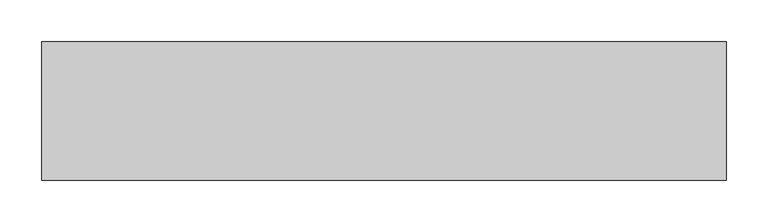
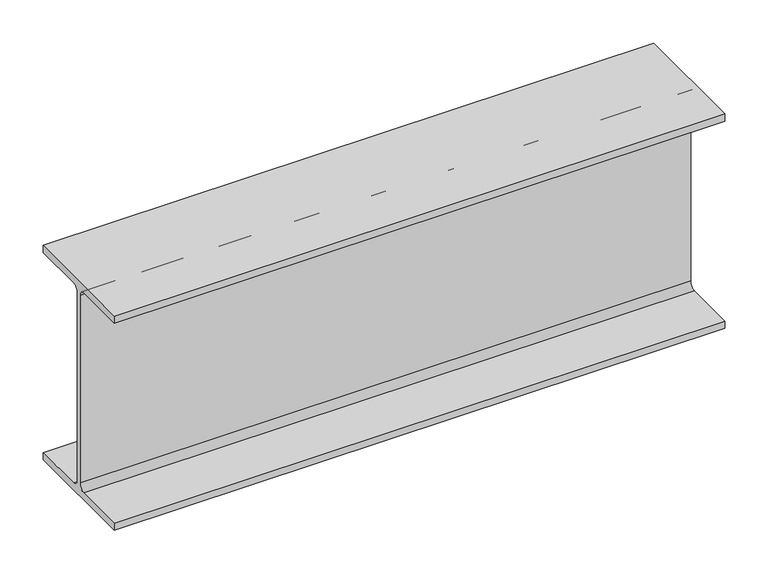
"""IFC4 building model written with IfcOpenShell, lengths in millimetres: beam geometry, Old_Steel Beam_H-KSD3502 : H_SB_ASB_H-390×300x10x16."""

import ifcopenshell
import ifcopenshell.guid

model = None  # the IFC model being written
_history = None  # IfcOwnerHistory: only IFC2X3 demands one
_inside = {}  # id of a spatial element -> (the spatial element, [elements in it])
_under = {}  # id of a project, library or spatial element -> (it, [spatial elements below it])
_declared = {}  # id of a project -> (the project, [libraries it declares])
_typed = {}  # id of a type object -> (the type object, [elements of that type])
_made_of = {}  # id of a material, layer set ... -> (it, [elements and type objects made of it])


def new_model(schema):
    """Start an empty IFC model of exactly this schema.

    Asked for "IFC4X3", IfcOpenShell would pick the latest addendum, in which some entities
    have other attributes; the version numbers below select the first issue.
    IFC2X3 requires an IfcOwnerHistory on every rooted entity: one is made here for all.
    """
    global model, _history
    if schema == "IFC4X3":
        model = ifcopenshell.file(schema_version=(4, 3, 0, 0))
    else:
        model = ifcopenshell.file(schema=schema)
    _inside.clear()
    _under.clear()
    _declared.clear()
    _typed.clear()
    _made_of.clear()
    _history = None
    if model.schema == "IFC2X3":
        org = make("IfcOrganization", Name="unknown")
        user = make(
            "IfcPersonAndOrganization",
            ThePerson=make("IfcPerson", FamilyName="unknown"),
            TheOrganization=org,
        )
        app = make(
            "IfcApplication",
            ApplicationDeveloper=org,
            Version="unknown",
            ApplicationFullName="unknown",
            ApplicationIdentifier="unknown",
        )
        _history = make(
            "IfcOwnerHistory",
            OwningUser=user,
            OwningApplication=app,
            ChangeAction="ADDED",
            CreationDate=0,
        )
    return model


def make(cls, **values):
    """One entity of the class cls with the attributes given. An attribute that is None is left unset."""
    return model.create_entity(
        cls, **{name: value for name, value in values.items() if value is not None}
    )


def rooted(cls, **values):
    """An entity with a GlobalId (a new one), such as an element, a storey or a relation."""
    return make(cls, GlobalId=ifcopenshell.guid.new(), OwnerHistory=_history, **values)


def si_unit(unit_type, name, prefix=None):
    """IfcSIUnit, for example si_unit("LENGTHUNIT", "METRE", prefix="MILLI")."""
    return make("IfcSIUnit", UnitType=unit_type, Prefix=prefix, Name=name)


def assignment(units):
    """IfcUnitAssignment: the units of a project."""
    return None if units is None else make("IfcUnitAssignment", Units=units)


def point(xyz):
    """IfcCartesianPoint."""
    return None if xyz is None else make("IfcCartesianPoint", Coordinates=xyz)


def direction(xyz):
    """IfcDirection."""
    return None if xyz is None else make("IfcDirection", DirectionRatios=xyz)


def frame(location, z_axis=None, x_axis=None):
    """IfcAxis2Placement3D, a coordinate frame: its origin and axes. An axis left out is left unset."""
    return make(
        "IfcAxis2Placement3D",
        Location=point(location),
        Axis=direction(z_axis),
        RefDirection=direction(x_axis),
    )


def frame_2d(location, x_axis=None):
    """IfcAxis2Placement2D, a coordinate frame in the plane: its origin and x axis."""
    return make(
        "IfcAxis2Placement2D", Location=point(location), RefDirection=direction(x_axis)
    )


def origin():
    """The frame at (0, 0, 0) with its axes left unset."""
    return frame((0.0, 0.0, 0.0))


def place(relative_to, where):
    """IfcLocalPlacement: puts the frame where relative to a parent placement (None: the world)."""
    return make(
        "IfcLocalPlacement", PlacementRelTo=relative_to, RelativePlacement=where
    )


def context(
    kind, dimensions, precision=None, world=None, true_north=None, identifier=None
):
    """IfcGeometricRepresentationContext, for example the 3D "Model" context."""
    return make(
        "IfcGeometricRepresentationContext",
        ContextIdentifier=identifier,
        ContextType=kind,
        CoordinateSpaceDimension=dimensions,
        Precision=precision,
        WorldCoordinateSystem=world,
        TrueNorth=true_north,
    )


def project(units=None, contexts=None):
    """IfcProject with its units and contexts."""
    return rooted(
        "IfcProject",
        Name="project",
        RepresentationContexts=contexts,
        UnitsInContext=assignment(units),
    )


def spatial(cls, under=None, at=None, **own):
    """A site, building, storey or space (cls), placed at a placement, below another one or the project."""
    s = rooted(cls, ObjectPlacement=at, **own)
    if under is not None:
        _under.setdefault(under.id(), (under, []))[1].append(s)
    return s


def polyline(points):
    """IfcPolyline through the points."""
    return make("IfcPolyline", Points=[point(p) for p in points])


def circle_curve(where, radius):
    """IfcCircle in the frame where."""
    return make("IfcCircle", Position=where, Radius=radius)


def trimmed(basis, trim1, trim2, sense, master):
    """IfcTrimmedCurve: the piece of a basis curve between two trims."""
    return make(
        "IfcTrimmedCurve",
        BasisCurve=basis,
        Trim1=trim1,
        Trim2=trim2,
        SenseAgreement=sense,
        MasterRepresentation=master,
    )


def segment(curve, same_sense, transition):
    """IfcCompositeCurveSegment."""
    return make(
        "IfcCompositeCurveSegment",
        Transition=transition,
        SameSense=same_sense,
        ParentCurve=curve,
    )


def composite_curve(segments, self_intersect=None):
    """IfcCompositeCurve: segments joined end to end."""
    return make("IfcCompositeCurve", Segments=segments, SelfIntersect=self_intersect)


def outline(outer, holes=None, kind="AREA"):
    """IfcArbitraryClosedProfileDef: a profile drawn as a closed curve; with holes, ...WithVoids."""
    if holes is None:
        return make("IfcArbitraryClosedProfileDef", ProfileType=kind, OuterCurve=outer)
    return make(
        "IfcArbitraryProfileDefWithVoids",
        ProfileType=kind,
        OuterCurve=outer,
        InnerCurves=holes,
    )


def extrude(swept, where, along, depth):
    """IfcExtrudedAreaSolid: the profile swept, set in the frame where, extruded along a direction by depth."""
    return make(
        "IfcExtrudedAreaSolid",
        SweptArea=swept,
        Position=where,
        ExtrudedDirection=direction(along),
        Depth=depth,
    )


def shape(context_of_items, identifier, shape_type, items):
    """IfcShapeRepresentation: the items that make up one representation, for example the "Body"."""
    return make(
        "IfcShapeRepresentation",
        ContextOfItems=context_of_items,
        RepresentationIdentifier=identifier,
        RepresentationType=shape_type,
        Items=items,
    )


def source(mapping_origin, context_of_items, identifier, shape_type, items):
    """IfcRepresentationMap: a shape defined once, which mapped items show again and again."""
    return make(
        "IfcRepresentationMap",
        MappingOrigin=mapping_origin,
        MappedRepresentation=shape(context_of_items, identifier, shape_type, items),
    )


def transform(
    local_origin,
    x_axis=None,
    y_axis=None,
    z_axis=None,
    scale=None,
    scale2=None,
    scale3=None,
    uniform=True,
):
    """IfcCartesianTransformationOperator3D, or its non-uniform kind. x_axis, y_axis, z_axis: its Axis1, 2, 3."""
    if uniform:
        return make(
            "IfcCartesianTransformationOperator3D",
            Axis1=direction(x_axis),
            Axis2=direction(y_axis),
            LocalOrigin=point(local_origin),
            Scale=scale,
            Axis3=direction(z_axis),
        )
    return make(
        "IfcCartesianTransformationOperator3DnonUniform",
        Axis1=direction(x_axis),
        Axis2=direction(y_axis),
        LocalOrigin=point(local_origin),
        Scale=scale,
        Axis3=direction(z_axis),
        Scale2=scale2,
        Scale3=scale3,
    )


def mapped(mapping_source, mapping_target):
    """IfcMappedItem: shows the shape of a source again, moved by a transform."""
    return make(
        "IfcMappedItem", MappingSource=mapping_source, MappingTarget=mapping_target
    )


def made_of(thing, what):
    """Note that an element or type object is made of a material, layer set ...; save() writes the relation."""
    if what is not None:
        _made_of.setdefault(what.id(), (what, []))[1].append(thing)
    return thing


def element(
    cls,
    number,
    at=None,
    inside=None,
    cuts=None,
    type_object=None,
    material=None,
    context=None,
    identifier="Body",
    shape_type=None,
    held_by="IfcProductDefinitionShape",
    body=None,
    shapes=None,
    **own,
):
    """One element of the class cls, such as IfcWall. Its Tag is "e" and its number.

    at: its placement. inside: the storey or other place that contains it. cuts: it is an
    opening in that element (IfcRelVoidsElement). A single representation is given by context,
    identifier, shape_type and body (its items); several are given by shapes. held_by: the class
    of the entity that holds the representations. save() writes the other relations.
    """
    e = rooted(cls, Tag="e%d" % number, ObjectPlacement=at, **own)
    if body is not None:
        shapes = [shape(context, identifier, shape_type, body)]
    if shapes is not None:
        e.Representation = make(held_by, Representations=shapes)
    if inside is not None:
        _inside.setdefault(inside.id(), (inside, []))[1].append(e)
    if cuts is not None:
        rooted(
            "IfcRelVoidsElement", RelatingBuildingElement=cuts, RelatedOpeningElement=e
        )
    if type_object is not None:
        _typed.setdefault(type_object.id(), (type_object, []))[1].append(e)
    return made_of(e, material)


def aggregate(whole, parts):
    """IfcRelAggregates: a whole, such as a stair, and the parts it consists of."""
    return rooted("IfcRelAggregates", RelatingObject=whole, RelatedObjects=parts)


def save(model, path):
    """Write the relations noted so far, then the file.

    IfcRelAggregates (storeys below a building ...), IfcRelContainedInSpatialStructure (elements
    in a storey), IfcRelDefinesByType, IfcRelAssociatesMaterial and IfcRelDeclares: one each for
    every whole, place, type object, material and project.
    """
    for whole, parts in _under.values():
        aggregate(whole, parts)
    for where, things in _inside.values():
        rooted(
            "IfcRelContainedInSpatialStructure",
            RelatedElements=things,
            RelatingStructure=where,
        )
    for kind, things in _typed.values():
        rooted("IfcRelDefinesByType", RelatedObjects=things, RelatingType=kind)
    for what, things in _made_of.values():
        rooted("IfcRelAssociatesMaterial", RelatedObjects=things, RelatingMaterial=what)
    for by, libraries in _declared.values():
        rooted("IfcRelDeclares", RelatingContext=by, RelatedDefinitions=libraries)
    model.write(path)


def beam_d0298337(model_context):
    return source(origin(), model_context, "Body", "SweptSolid", [
        extrude(outline(composite_curve([segment(polyline([(82.5, -141.5), (82.5, -151.7), (-82.5, -151.7), (-82.5, -141.5), (-11.9, -141.5)]), True, "CONTINUOUS"), segment(trimmed(circle_curve(frame_2d((-11.9, -132.6)), 8.9), [point((-11.9, -141.5))], [point((-3.0, -132.6))], True, "CARTESIAN"), True, "CONTINUOUS"), segment(polyline([(-3.0, -132.6), (-3.0, 132.6)]), True, "CONTINUOUS"), segment(trimmed(circle_curve(frame_2d((-11.9, 132.6)), 8.9), [point((-3.0, 132.6))], [point((-11.9, 141.5))], True, "CARTESIAN"), True, "CONTINUOUS"), segment(polyline([(-11.9, 141.5), (-82.5, 141.5), (-82.5, 151.7), (82.5, 151.7), (82.5, 141.5), (11.9, 141.5)]), True, "CONTINUOUS"), segment(trimmed(circle_curve(frame_2d((11.9, 132.6)), 8.9), [point((11.9, 141.5))], [point((3.0, 132.6))], True, "CARTESIAN"), True, "CONTINUOUS"), segment(polyline([(3.0, 132.6), (3.0, -132.6)]), True, "CONTINUOUS"), segment(trimmed(circle_curve(frame_2d((11.9, -132.6)), 8.9), [point((3.0, -132.6))], [point((11.9, -141.5))], True, "CARTESIAN"), True, "CONTINUOUS"), segment(polyline([(11.9, -141.5), (82.5, -141.5)]), True, "CONTINUOUS")], self_intersect=False)), frame((-402.2999994, 0.0, 0.0), z_axis=(1.0, 0.0, 0.0), x_axis=(0.0, 1.0, 0.0)), (0.0, 0.0, 1.0), 817.2999994),
    ])


if __name__ == "__main__":
    model = new_model("IFC4")
    model_context = context("Model", 3, world=origin())
    ifc_project = project(units=[si_unit("LENGTHUNIT", "METRE", prefix="MILLI")], contexts=[model_context])
    site = spatial("IfcSite", under=ifc_project)
    building = spatial("IfcBuilding", under=site)
    placement = place(None, origin())
    beam_shape = beam_d0298337(model_context)
    element("IfcBeam", 1, ObjectType="Old_Steel Beam_H-KSD3502 : H_SB_ASB_H-390×300x10x16", at=placement, inside=building, context=model_context, shape_type="MappedRepresentation", body=[
        mapped(beam_shape, transform((0.0, 0.0, 0.0), x_axis=(1.0, 0.0, 0.0), y_axis=(0.0, 1.0, 0.0), z_axis=(0.0, 0.0, 1.0))),
    ])
    save(model, "model.ifc")

# Revit data of these elements
# Type "Old_Steel Beam_H-KSD3502 : H_SB_ASB_H-390×300x10x16"
#   Width = 30.0 cm
#   Web Thickness = 1.0 cm
#   Web Fillet = 2.2 cm
#   Warping Constant = 2517770.0 cm⁶
#   Torsional Moment of Inertia = 94.3867 cm⁴
#   Torsional Modulus = 1.0 cm³
#   Section Area = 136.0 cm²
#   Plastic Modulus weak axis = 733.0 cm³
#   Plastic Modulus strong axis = 2190.0 cm³
#   Perimeter = 1.92 m²/m
#   Nominal Weight = 107.00 kgf/m
#   Moment of Inertia weak axis = 7210.00 cm⁴
#   Moment of Inertia strong axis = 38700.00 cm⁴
#   Height = 39.0 cm
#   Flange Thickness = 1.6 cm
#   Elastic Modulus weak axis = 481.0 cm³
#   Elastic Modulus strong axis = 1980.0 cm³
#   Centroid Vertical = 19.5 cm
#   Centroid Horizontal = 15.0 cm
#   Length [instance default] = 1.5240 m
#   Structural Material [instance default] = Steel, 45-345
#   Assembly Code = ""
# Element 1 (IfcBeam, "Old_Steel Beam_H-KSD3502 : H_SB_ASB_H-390×300x10x16")
#   Structural Material = none
# Materials
#   "Steel, 45-345": class "Metal", colour RGB 189 187 185, transparency 0, Description = "Steel 345 MPa", Cost = 0
